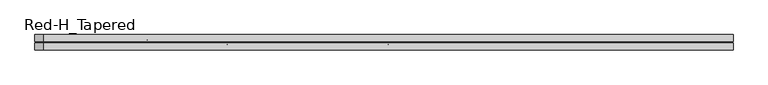
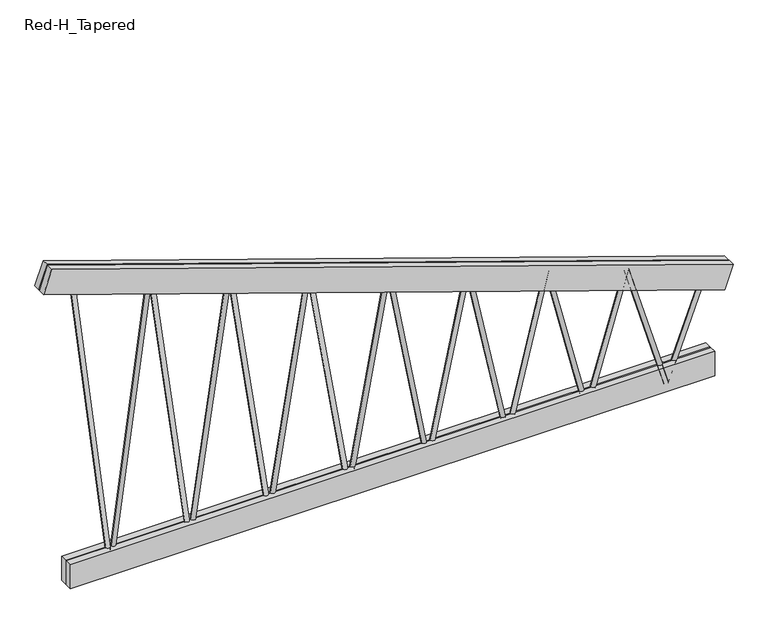
"""IFC4 building model written with IfcOpenShell, lengths in millimetres: beam geometry, Construction_Frames_RedBuilt_Openweb_Red-H_Tapered : Red-H_Tapered."""

import ifcopenshell
import ifcopenshell.guid

model = None  # the IFC model being written
_history = None  # IfcOwnerHistory: only IFC2X3 demands one
_inside = {}  # id of a spatial element -> (the spatial element, [elements in it])
_under = {}  # id of a project, library or spatial element -> (it, [spatial elements below it])
_declared = {}  # id of a project -> (the project, [libraries it declares])
_typed = {}  # id of a type object -> (the type object, [elements of that type])
_made_of = {}  # id of a material, layer set ... -> (it, [elements and type objects made of it])


def new_model(schema):
    """Start an empty IFC model of exactly this schema.

    Asked for "IFC4X3", IfcOpenShell would pick the latest addendum, in which some entities
    have other attributes; the version numbers below select the first issue.
    IFC2X3 requires an IfcOwnerHistory on every rooted entity: one is made here for all.
    """
    global model, _history
    if schema == "IFC4X3":
        model = ifcopenshell.file(schema_version=(4, 3, 0, 0))
    else:
        model = ifcopenshell.file(schema=schema)
    _inside.clear()
    _under.clear()
    _declared.clear()
    _typed.clear()
    _made_of.clear()
    _history = None
    if model.schema == "IFC2X3":
        org = make("IfcOrganization", Name="unknown")
        user = make(
            "IfcPersonAndOrganization",
            ThePerson=make("IfcPerson", FamilyName="unknown"),
            TheOrganization=org,
        )
        app = make(
            "IfcApplication",
            ApplicationDeveloper=org,
            Version="unknown",
            ApplicationFullName="unknown",
            ApplicationIdentifier="unknown",
        )
        _history = make(
            "IfcOwnerHistory",
            OwningUser=user,
            OwningApplication=app,
            ChangeAction="ADDED",
            CreationDate=0,
        )
    return model


def make(cls, **values):
    """One entity of the class cls with the attributes given. An attribute that is None is left unset."""
    return model.create_entity(
        cls, **{name: value for name, value in values.items() if value is not None}
    )


def rooted(cls, **values):
    """An entity with a GlobalId (a new one), such as an element, a storey or a relation."""
    return make(cls, GlobalId=ifcopenshell.guid.new(), OwnerHistory=_history, **values)


def si_unit(unit_type, name, prefix=None):
    """IfcSIUnit, for example si_unit("LENGTHUNIT", "METRE", prefix="MILLI")."""
    return make("IfcSIUnit", UnitType=unit_type, Prefix=prefix, Name=name)


def assignment(units):
    """IfcUnitAssignment: the units of a project."""
    return None if units is None else make("IfcUnitAssignment", Units=units)


def point(xyz):
    """IfcCartesianPoint."""
    return None if xyz is None else make("IfcCartesianPoint", Coordinates=xyz)


def direction(xyz):
    """IfcDirection."""
    return None if xyz is None else make("IfcDirection", DirectionRatios=xyz)


def frame(location, z_axis=None, x_axis=None):
    """IfcAxis2Placement3D, a coordinate frame: its origin and axes. An axis left out is left unset."""
    return make(
        "IfcAxis2Placement3D",
        Location=point(location),
        Axis=direction(z_axis),
        RefDirection=direction(x_axis),
    )


def frame_2d(location, x_axis=None):
    """IfcAxis2Placement2D, a coordinate frame in the plane: its origin and x axis."""
    return make(
        "IfcAxis2Placement2D", Location=point(location), RefDirection=direction(x_axis)
    )


def origin():
    """The frame at (0, 0, 0) with its axes left unset."""
    return frame((0.0, 0.0, 0.0))


def origin_2d():
    """The frame at (0, 0) in the plane with its x axis left unset."""
    return frame_2d((0.0, 0.0))


def place(relative_to, where):
    """IfcLocalPlacement: puts the frame where relative to a parent placement (None: the world)."""
    return make(
        "IfcLocalPlacement", PlacementRelTo=relative_to, RelativePlacement=where
    )


def context(
    kind, dimensions, precision=None, world=None, true_north=None, identifier=None
):
    """IfcGeometricRepresentationContext, for example the 3D "Model" context."""
    return make(
        "IfcGeometricRepresentationContext",
        ContextIdentifier=identifier,
        ContextType=kind,
        CoordinateSpaceDimension=dimensions,
        Precision=precision,
        WorldCoordinateSystem=world,
        TrueNorth=true_north,
    )


def project(units=None, contexts=None):
    """IfcProject with its units and contexts."""
    return rooted(
        "IfcProject",
        Name="project",
        RepresentationContexts=contexts,
        UnitsInContext=assignment(units),
    )


def spatial(cls, under=None, at=None, **own):
    """A site, building, storey or space (cls), placed at a placement, below another one or the project."""
    s = rooted(cls, ObjectPlacement=at, **own)
    if under is not None:
        _under.setdefault(under.id(), (under, []))[1].append(s)
    return s


def polyline(points):
    """IfcPolyline through the points."""
    return make("IfcPolyline", Points=[point(p) for p in points])


def circle_curve(where, radius):
    """IfcCircle in the frame where."""
    return make("IfcCircle", Position=where, Radius=radius)


def trimmed(basis, trim1, trim2, sense, master):
    """IfcTrimmedCurve: the piece of a basis curve between two trims."""
    return make(
        "IfcTrimmedCurve",
        BasisCurve=basis,
        Trim1=trim1,
        Trim2=trim2,
        SenseAgreement=sense,
        MasterRepresentation=master,
    )


def segment(curve, same_sense, transition):
    """IfcCompositeCurveSegment."""
    return make(
        "IfcCompositeCurveSegment",
        Transition=transition,
        SameSense=same_sense,
        ParentCurve=curve,
    )


def composite_curve(segments, self_intersect=None):
    """IfcCompositeCurve: segments joined end to end."""
    return make("IfcCompositeCurve", Segments=segments, SelfIntersect=self_intersect)


def outline(outer, holes=None, kind="AREA"):
    """IfcArbitraryClosedProfileDef: a profile drawn as a closed curve; with holes, ...WithVoids."""
    if holes is None:
        return make("IfcArbitraryClosedProfileDef", ProfileType=kind, OuterCurve=outer)
    return make(
        "IfcArbitraryProfileDefWithVoids",
        ProfileType=kind,
        OuterCurve=outer,
        InnerCurves=holes,
    )


def extrude(swept, where, along, depth):
    """IfcExtrudedAreaSolid: the profile swept, set in the frame where, extruded along a direction by depth."""
    return make(
        "IfcExtrudedAreaSolid",
        SweptArea=swept,
        Position=where,
        ExtrudedDirection=direction(along),
        Depth=depth,
    )


def shape(context_of_items, identifier, shape_type, items):
    """IfcShapeRepresentation: the items that make up one representation, for example the "Body"."""
    return make(
        "IfcShapeRepresentation",
        ContextOfItems=context_of_items,
        RepresentationIdentifier=identifier,
        RepresentationType=shape_type,
        Items=items,
    )


def source(mapping_origin, context_of_items, identifier, shape_type, items):
    """IfcRepresentationMap: a shape defined once, which mapped items show again and again."""
    return make(
        "IfcRepresentationMap",
        MappingOrigin=mapping_origin,
        MappedRepresentation=shape(context_of_items, identifier, shape_type, items),
    )


def transform(
    local_origin,
    x_axis=None,
    y_axis=None,
    z_axis=None,
    scale=None,
    scale2=None,
    scale3=None,
    uniform=True,
):
    """IfcCartesianTransformationOperator3D, or its non-uniform kind. x_axis, y_axis, z_axis: its Axis1, 2, 3."""
    if uniform:
        return make(
            "IfcCartesianTransformationOperator3D",
            Axis1=direction(x_axis),
            Axis2=direction(y_axis),
            LocalOrigin=point(local_origin),
            Scale=scale,
            Axis3=direction(z_axis),
        )
    return make(
        "IfcCartesianTransformationOperator3DnonUniform",
        Axis1=direction(x_axis),
        Axis2=direction(y_axis),
        LocalOrigin=point(local_origin),
        Scale=scale,
        Axis3=direction(z_axis),
        Scale2=scale2,
        Scale3=scale3,
    )


def mapped(mapping_source, mapping_target):
    """IfcMappedItem: shows the shape of a source again, moved by a transform."""
    return make(
        "IfcMappedItem", MappingSource=mapping_source, MappingTarget=mapping_target
    )


def made_of(thing, what):
    """Note that an element or type object is made of a material, layer set ...; save() writes the relation."""
    if what is not None:
        _made_of.setdefault(what.id(), (what, []))[1].append(thing)
    return thing


def element(
    cls,
    number,
    at=None,
    inside=None,
    cuts=None,
    type_object=None,
    material=None,
    context=None,
    identifier="Body",
    shape_type=None,
    held_by="IfcProductDefinitionShape",
    body=None,
    shapes=None,
    **own,
):
    """One element of the class cls, such as IfcWall. Its Tag is "e" and its number.

    at: its placement. inside: the storey or other place that contains it. cuts: it is an
    opening in that element (IfcRelVoidsElement). A single representation is given by context,
    identifier, shape_type and body (its items); several are given by shapes. held_by: the class
    of the entity that holds the representations. save() writes the other relations.
    """
    e = rooted(cls, Tag="e%d" % number, ObjectPlacement=at, **own)
    if body is not None:
        shapes = [shape(context, identifier, shape_type, body)]
    if shapes is not None:
        e.Representation = make(held_by, Representations=shapes)
    if inside is not None:
        _inside.setdefault(inside.id(), (inside, []))[1].append(e)
    if cuts is not None:
        rooted(
            "IfcRelVoidsElement", RelatingBuildingElement=cuts, RelatedOpeningElement=e
        )
    if type_object is not None:
        _typed.setdefault(type_object.id(), (type_object, []))[1].append(e)
    return made_of(e, material)


def aggregate(whole, parts):
    """IfcRelAggregates: a whole, such as a stair, and the parts it consists of."""
    return rooted("IfcRelAggregates", RelatingObject=whole, RelatedObjects=parts)


def save(model, path):
    """Write the relations noted so far, then the file.

    IfcRelAggregates (storeys below a building ...), IfcRelContainedInSpatialStructure (elements
    in a storey), IfcRelDefinesByType, IfcRelAssociatesMaterial and IfcRelDeclares: one each for
    every whole, place, type object, material and project.
    """
    for whole, parts in _under.values():
        aggregate(whole, parts)
    for where, things in _inside.values():
        rooted(
            "IfcRelContainedInSpatialStructure",
            RelatedElements=things,
            RelatingStructure=where,
        )
    for kind, things in _typed.values():
        rooted("IfcRelDefinesByType", RelatedObjects=things, RelatingType=kind)
    for what, things in _made_of.values():
        rooted("IfcRelAssociatesMaterial", RelatedObjects=things, RelatingMaterial=what)
    for by, libraries in _declared.values():
        rooted("IfcRelDeclares", RelatingContext=by, RelatedDefinitions=libraries)
    model.write(path)


def red_h_tapered_d2c9fe49(model_context):
    return source(origin(), model_context, "Body", "SweptSolid", [
        extrude(outline(composite_curve([segment(trimmed(circle_curve(origin_2d(), 12.7), [point((0.0, 12.7))], [point((0.0, -12.7000001))], False, "CARTESIAN"), True, "CONTINUOUS"), segment(trimmed(circle_curve(origin_2d(), 12.7), [point((0.0, -12.7000001))], [point((0.0, 12.7))], False, "CARTESIAN"), True, "CONTINUOUS")], self_intersect=False)), frame((-217.9835937, 0.0, -367.0101562), z_axis=(-0.16059437505424784, 0.0, 0.9870204895041114), x_axis=(0.0, -1.0, 0.0)), (0.0, 0.0, 1.0), 1357.3550984),
        extrude(outline(composite_curve([segment(trimmed(circle_curve(origin_2d(), 12.7), [point((0.0, -12.7000001))], [point((0.0, 12.7))], False, "CARTESIAN"), True, "CONTINUOUS"), segment(trimmed(circle_curve(origin_2d(), 12.7), [point((0.0, 12.7))], [point((0.0, -12.7000001))], False, "CARTESIAN"), True, "CONTINUOUS")], self_intersect=False)), frame((-653.9507812, 0.0, -367.0101562), z_axis=(0.16059437505424665, 0.0, 0.9870204895041117), x_axis=(0.0, -1.0, 0.0)), (0.0, 0.0, 1.0), 1357.3550984),
        extrude(outline(composite_curve([segment(trimmed(circle_curve(origin_2d(), 12.7), [point((0.0, 12.7))], [point((0.0, -12.7000001))], False, "CARTESIAN"), True, "CONTINUOUS"), segment(trimmed(circle_curve(origin_2d(), 12.7), [point((0.0, -12.7000001))], [point((0.0, 12.7))], False, "CARTESIAN"), True, "CONTINUOUS")], self_intersect=False)), frame((-653.9507812, 0.0, -367.0101562), z_axis=(-0.14467649318910314, 0.0, 0.9894790105497455), x_axis=(0.0, -1.0, 0.0)), (0.0, 0.0, 1.0), 1506.6966924),
        extrude(outline(composite_curve([segment(trimmed(circle_curve(origin_2d(), 12.7), [point((0.0, -12.7000001))], [point((0.0, 12.7))], False, "CARTESIAN"), True, "CONTINUOUS"), segment(trimmed(circle_curve(origin_2d(), 12.7), [point((0.0, 12.7))], [point((0.0, -12.7000001))], False, "CARTESIAN"), True, "CONTINUOUS")], self_intersect=False)), frame((-1089.9179687, 0.0, -367.0101562), z_axis=(0.14467649318911152, 0.0, 0.9894790105497443), x_axis=(0.0, -1.0, 0.0)), (0.0, 0.0, 1.0), 1506.6966924),
        extrude(outline(composite_curve([segment(trimmed(circle_curve(origin_2d(), 12.7), [point((0.0, 12.7))], [point((0.0, -12.7000001))], False, "CARTESIAN"), True, "CONTINUOUS"), segment(trimmed(circle_curve(origin_2d(), 12.7), [point((0.0, -12.7000001))], [point((0.0, 12.7))], False, "CARTESIAN"), True, "CONTINUOUS")], self_intersect=False)), frame((-1089.9179687, 0.0, -367.0101562), z_axis=(-0.1316041042225624, 0.0, 0.9913023553647883), x_axis=(0.0, -1.0, 0.0)), (0.0, 0.0, 1.0), 1656.3586298),
        extrude(outline(composite_curve([segment(trimmed(circle_curve(origin_2d(), 12.7), [point((0.0, -12.7000001))], [point((0.0, 12.7))], False, "CARTESIAN"), True, "CONTINUOUS"), segment(trimmed(circle_curve(origin_2d(), 12.7), [point((0.0, 12.7))], [point((0.0, -12.7000001))], False, "CARTESIAN"), True, "CONTINUOUS")], self_intersect=False)), frame((-1525.8851562, 0.0, -367.0101562), z_axis=(0.13160410422255567, 0.0, 0.9913023553647892), x_axis=(0.0, -1.0, 0.0)), (0.0, 0.0, 1.0), 1656.3586298),
        extrude(outline(composite_curve([segment(trimmed(circle_curve(origin_2d(), 12.7), [point((0.0, 12.6999999))], [point((0.0, -12.7))], False, "CARTESIAN"), True, "CONTINUOUS"), segment(trimmed(circle_curve(origin_2d(), 12.7), [point((0.0, -12.7))], [point((0.0, 12.6999999))], False, "CARTESIAN"), True, "CONTINUOUS")], self_intersect=False)), frame((-1525.8851562, 0.0, -367.0101562), z_axis=(-0.12068220454190359, 0.0, 0.9926911934266901), x_axis=(0.0, -1.0, 0.0)), (0.0, 0.0, 1.0), 1806.2612842),
        extrude(outline(composite_curve([segment(trimmed(circle_curve(origin_2d(), 12.7), [point((0.0, 12.7000001))], [point((0.0, -12.7))], False, "CARTESIAN"), True, "CONTINUOUS"), segment(trimmed(circle_curve(origin_2d(), 12.7), [point((0.0, -12.7))], [point((0.0, 12.7000001))], False, "CARTESIAN"), True, "CONTINUOUS")], self_intersect=False)), frame((1525.8851562, 0.0, -367.0101562), z_axis=(0.3495884350369082, 0.0, 0.9369033707317129), x_axis=(0.0, -1.0, 0.0)), (0.0, 0.0, 1.0), 623.5434926),
        extrude(outline(composite_curve([segment(trimmed(circle_curve(origin_2d(), 12.7), [point((0.0, -12.6999999))], [point((0.0, 12.7))], False, "CARTESIAN"), True, "CONTINUOUS"), segment(trimmed(circle_curve(origin_2d(), 12.7), [point((0.0, 12.7))], [point((0.0, -12.6999999))], False, "CARTESIAN"), True, "CONTINUOUS")], self_intersect=False)), frame((1525.8851562, 0.0, -367.0101562), z_axis=(-0.28422583294581855, 0.0, 0.9587573602774874), x_axis=(0.0, -1.0, 0.0)), (0.0, 0.0, 1.0), 766.9380066),
        extrude(outline(composite_curve([segment(trimmed(circle_curve(origin_2d(), 12.7), [point((0.0, 12.7))], [point((0.0, -12.6999999))], False, "CARTESIAN"), True, "CONTINUOUS"), segment(trimmed(circle_curve(origin_2d(), 12.7), [point((0.0, -12.6999999))], [point((0.0, 12.7))], False, "CARTESIAN"), True, "CONTINUOUS")], self_intersect=False)), frame((1089.9179687, 0.0, -367.0101562), z_axis=(0.2842258329458186, 0.0, 0.9587573602774874), x_axis=(0.0, -1.0, 0.0)), (0.0, 0.0, 1.0), 766.9380066),
        extrude(outline(composite_curve([segment(trimmed(circle_curve(origin_2d(), 12.7), [point((0.0, -12.6999999))], [point((0.0, 12.7))], False, "CARTESIAN"), True, "CONTINUOUS"), segment(trimmed(circle_curve(origin_2d(), 12.7), [point((0.0, 12.7))], [point((0.0, -12.6999999))], False, "CARTESIAN"), True, "CONTINUOUS")], self_intersect=False)), frame((1089.9179687, 0.0, -367.0101562), z_axis=(-0.2388012536077187, 0.0, 0.9710684637425839), x_axis=(0.0, -1.0, 0.0)), (0.0, 0.0, 1.0), 912.8243276),
        extrude(outline(composite_curve([segment(trimmed(circle_curve(origin_2d(), 12.7), [point((0.0, 12.7))], [point((0.0, -12.6999999))], False, "CARTESIAN"), True, "CONTINUOUS"), segment(trimmed(circle_curve(origin_2d(), 12.7), [point((0.0, -12.6999999))], [point((0.0, 12.7))], False, "CARTESIAN"), True, "CONTINUOUS")], self_intersect=False)), frame((653.9507812, 0.0, -367.0101562), z_axis=(0.2388012536077183, 0.0, 0.971068463742584), x_axis=(0.0, -1.0, 0.0)), (0.0, 0.0, 1.0), 912.8243276),
        extrude(outline(composite_curve([segment(trimmed(circle_curve(origin_2d(), 12.7), [point((0.0, -12.7))], [point((0.0, 12.7000001))], False, "CARTESIAN"), True, "CONTINUOUS"), segment(trimmed(circle_curve(origin_2d(), 12.7), [point((0.0, 12.7000001))], [point((0.0, -12.7))], False, "CARTESIAN"), True, "CONTINUOUS")], self_intersect=False)), frame((653.9507812, 0.0, -367.0101562), z_axis=(-0.2056110919797595, 0.0, 0.9786337817870845), x_axis=(0.0, -1.0, 0.0)), (0.0, 0.0, 1.0), 1060.1742914),
        extrude(outline(composite_curve([segment(trimmed(circle_curve(origin_2d(), 12.7), [point((0.0, 12.7))], [point((0.0, -12.7000001))], False, "CARTESIAN"), True, "CONTINUOUS"), segment(trimmed(circle_curve(origin_2d(), 12.7), [point((0.0, -12.7000001))], [point((0.0, 12.7))], False, "CARTESIAN"), True, "CONTINUOUS")], self_intersect=False)), frame((217.9835938, 0.0, -367.0101562), z_axis=(0.20561109197976007, 0.0, 0.9786337817870844), x_axis=(0.0, -1.0, 0.0)), (0.0, 0.0, 1.0), 1060.1742914),
        extrude(outline(composite_curve([segment(trimmed(circle_curve(origin_2d(), 12.7), [point((0.0, -12.7))], [point((0.0, 12.6999999))], False, "CARTESIAN"), True, "CONTINUOUS"), segment(trimmed(circle_curve(origin_2d(), 12.7), [point((0.0, 12.6999999))], [point((0.0, -12.7))], False, "CARTESIAN"), True, "CONTINUOUS")], self_intersect=False)), frame((217.9835938, 0.0, -367.0101562), z_axis=(-0.1803824083648695, 0.0, 0.9835965569035353), x_axis=(0.0, -1.0, 0.0)), (0.0, 0.0, 1.0), 1208.4526187),
        extrude(outline(composite_curve([segment(trimmed(circle_curve(origin_2d(), 12.7), [point((0.0, -12.7))], [point((0.0, 12.6999999))], False, "CARTESIAN"), True, "CONTINUOUS"), segment(trimmed(circle_curve(origin_2d(), 12.7), [point((0.0, 12.6999999))], [point((0.0, -12.7))], False, "CARTESIAN"), True, "CONTINUOUS")], self_intersect=False)), frame((-217.9835937, 0.0, -367.0101562), z_axis=(0.18038240836484612, 0.0, 0.9835965569035395), x_axis=(0.0, -1.0, 0.0)), (0.0, 0.0, 1.0), 1208.4526187),
        extrude(outline(polyline([(-1769.26875, -41.275), (-1769.26875, -3.175), (1769.26875, -3.175), (1769.26875, -41.275), (-1769.26875, -41.275)])), frame((0.0, 0.0, -386.0601562), z_axis=(0.0, 0.0, 1.0), x_axis=(1.0, 0.0, 0.0)), (0.0, 0.0, 1.0), 139.7),
        extrude(outline(polyline([(-1769.26875, 3.175), (-1769.26875, 41.275), (1769.26875, 41.275), (1769.26875, 3.175), (-1769.26875, 3.175)])), frame((0.0, 0.0, -386.0601562), z_axis=(0.0, 0.0, 1.0), x_axis=(1.0, 0.0, 0.0)), (0.0, 0.0, 1.0), 139.7),
        extrude(outline(polyline([(0.0, -38.1), (0.0, 0.0), (3955.4922335, 0.0), (3955.4922335, -38.1), (0.0, -38.1)])), frame((-1916.1711244, -3.175, 1374.0892294), z_axis=(0.3242832811430626, 0.0, 0.9459600168987532), x_axis=(0.9459600168987532, 0.0, -0.3242832811430626)), (0.0, 0.0, 1.0), 139.7),
        extrude(outline(polyline([(0.0, -38.1), (0.0, 0.0), (3955.4922335, 0.0), (3955.4922335, -38.1), (0.0, -38.1)])), frame((-1916.1711244, 41.275, 1374.0892294), z_axis=(0.3242832811430624, 0.0, 0.9459600168987533), x_axis=(0.9459600168987533, 0.0, -0.3242832811430624)), (0.0, 0.0, 1.0), 139.7),
    ])


if __name__ == "__main__":
    model = new_model("IFC4")
    model_context = context("Model", 3, world=origin())
    ifc_project = project(units=[si_unit("LENGTHUNIT", "METRE", prefix="MILLI")], contexts=[model_context])
    site = spatial("IfcSite", under=ifc_project)
    building = spatial("IfcBuilding", under=site)
    placement = place(None, origin())
    red_h_tapered_shape = red_h_tapered_d2c9fe49(model_context)
    element("IfcBeam", 1, ObjectType="Construction_Frames_RedBuilt_Openweb_Red-H_Tapered : Red-H_Tapered", at=placement, inside=building, context=model_context, shape_type="MappedRepresentation", body=[
        mapped(red_h_tapered_shape, transform((0.0, 0.0, 0.0), x_axis=(1.0, 0.0, 0.0), y_axis=(0.0, 1.0, 0.0), z_axis=(0.0, 0.0, 1.0))),
    ])
    save(model, "model.ifc")

# Revit data of these elements
# Type "Construction_Frames_RedBuilt_Openweb_Red-H_Tapered : Red-H_Tapered"
#   Youtube clip = ""
#   Weight Net (Kg) = "0"
#   Webs = "Up to 2\" diameter tubular steel"
#   Uniformat II Description = ""
#   Uniformat II Code = ""
#   Uniclass 2015 Name = "Softwood trusses"
#   Uniclass 2015 Code = "Pr_20_85_90_81"
#   Uniclass 2.0 Description = "Structural Framing Systems"
#   Uniclass 2.0 Code = "SS-15-10-75"
#   Uniclass 1.4 Description = "Trusses"
#   Uniclass 1.4 Code = "L3523"
#   UNSPSC Code = "30103606"
#   Technical description = "http://www.redbuilt.com/reference/literature-and-other-resources"
#   Region South America = "None"
#   Region Oceania = "None"
#   Region North America = "US"
#   Region Middle East = "None"
#   Region Europe = "None"
#   Region Asia = "None"
#   Region Antarctica = "None"
#   Region Africa = "None"
#   QR code = "http://bimobject.com/redbuilt/product/redbuilt-0003"
#   Product url = "http://www.redbuilt.com/products/default.aspx?id=2"
#   Product group = "Wood Trusses"
#   Product family = "Construction"
#   Product data url = "https://bimobject.com/redbuilt/product/redbuilt-0003"
#   Product certification = ""
#   Product SKU = "redbuilt-0003"
#   Product Page URL = "http://www.redbuilt.com/commercial-systems/red-m-red-h-open-web-trusses"
#   Product Guid = "2c5793f2-6ffb-4665-b825-cf90c048e711"
#   Product Documentation Link = "http://www.redbuilt.com/documents/OW_Guide_2017_07_LowRes_wLinks.pdf"
#   OmniClass Description = "Wood Trusses"
#   OmniClass Code = "23-13 35 19 13 17"
#   NBS Reference Description = ""
#   NBS Reference Code = ""
#   Material secondary = "Steel"
#   Material main = "Wood"
#   Masterformat 2014 Description = "Metal-Web Wood Joists"
#   Masterformat 2014 Code = "06 17 36"
#   Manufacturer name = "RedBuilt"
#   Manufacturer country = "United States"
#   Installation instructions = "http://www.redbuilt.com/documents/Installation_Sheets_Open-Web.pdf"
#   IFC Classification = ""
#   EAN code = ""
#   Design country = "United States"
#   Product Information = "http://redbuilt.com/products/default.aspx?id=2"
#   Model = "Red-H-Tapered"
#   Manufacturer URL = "http://redbuilt.com/"
#   Manufacturer = "RedBuilt™"
#   Description = "Open Web Truss"
#   Date of publishing = "8/17/2010"
#   Contact us = "http://redbuilt.com/contact/"
#   Chords = "Double 1½\" x 5½\" MSR lumber"
#   COBIe Type Category = ""
#   Brand url = "http://www.redbuilt.com"
#   BIMobject main category code = "construction"
#   BIMobject main category = "Construction"
#   BIMobject category code = "construction-frames-trusses"
#   BIMobject category = "Frames & Trusses"
#   Web Radius = 0' - 0 1/2"
#   Web Layout Offset Start [instance default] = 0' - 5"
#   Web Layout Offset End [instance default] = 0' - 5"
#   Web Diameter = 0' - 1"
#   TotalLength [instance default] = 20' - 0"
#   Span Minimum = 4' - 0"
#   Span Maximum = 70' - 0"
#   Span Limit [instance default] = 20' - 0"
#   Nominal width = 0' - 0"
#   Nominal height = 0' - 0"
#   Inner Depth Top [instance default] = 0' - 2.76372"
#   Depth Start [instance default] = 6' - 0"
#   Top Chord Length [instance default] = 20' - 1.19701"
#   TC Extension Start Aux [instance default] = 0' - 0"
#   TC Extension End Aux [instance default] = 0' - 0"
#   T-B Chord Length Difference L [instance default] = 0' - 4"
#   T-B Chord Length Difference [instance default] = 0' - 4"
#   Height 2 [instance default] = 6' - 0"
#   Depth Minimum at Wall = 2' - 0"
#   Depth Maximum at Wall = 6' - 0"
#   Depth Lower End [instance default] = 2' - 0"
#   Depth Higher End [instance default] = 6' - 0"
#   Depth End [instance default] = 2' - 0"
#   Depth 2 [instance default] = 2' - 0"
#   Chord Width = 0' - 3 1/4"
#   Chord Thickness = 0' - 1 1/2"
#   Chord Depth = 0' - 5 1/2"
#   Offset Start [instance default] = 0' - 0"
#   TC Extension Start [instance default] = 0' - 0"
#   End Panel = 0' - 5"
#   Offset End [instance default] = 0' - 0"
#   TC Extension End [instance default] = 0' - 0"
#   Length [instance default] = 20' - 0"
#   Angle [instance default] = 5.71059°
#   Span Limit Warning [instance default] = no
#   Edition number = 1
#   Top Bearing Start [instance default] = yes
#   Top Bearing End [instance default] = yes
#   Bottom Bearing Start [instance default] = no
#   Bottom Bearing End [instance default] = no
#   8 Panels [instance default] = yes
#   16 Panels [instance default] = no
#   12 Panels [instance default] = no
#   Web Material = RedBuilt-Steel, Galvanized
#   Clip Material = RedBuilt-Steel, Galvanized
#   Chords Material = RedBuilt-MSR
#   URL = ""
#   Assembly Code = ""
# Element 1 (IfcBeam, "Construction_Frames_RedBuilt_Openweb_Red-H_Tapered : Red-H_Tapered")
#   TotalLength = 12' - 3 5/16"
#   Span Limit = 12' - 3 5/16"
#   Inner Depth Top = 0' - 2.9071"
#   Top Chord Length = 12' - 11.72804"
#   Depth 2 = 4' - 2 1/2"
#   Angle = 18.9222°
#   Materials on its faces: "RedBuilt-Steel, Galvanized", "RedBuilt-MSR"
# Materials
#   "RedBuilt-Steel, Galvanized": class "Metal", colour RGB 164 172 176, transparency 0, Manufacturer = "RedBuilt. LLC", Comments = "Openweb Metal Web", URL = "http://www.redbuilt.com/", Description = "Galvanized steel", Cost = 0
#   "RedBuilt-MSR": class "Wood", colour RGB 213 182 136, transparency 0, Manufacturer = "RedBuilt, LLC", URL = "http://www.redbuilt.com/", Cost = 0
